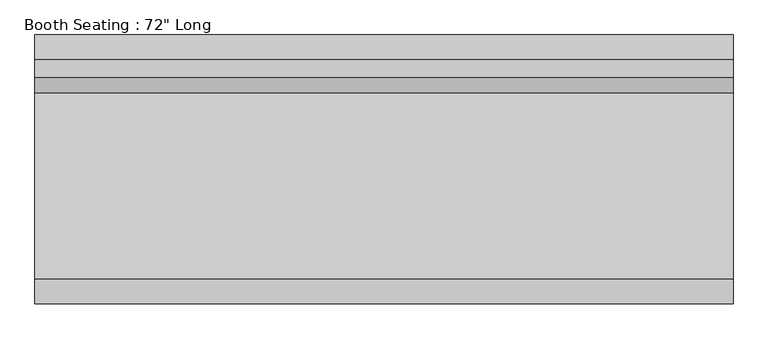
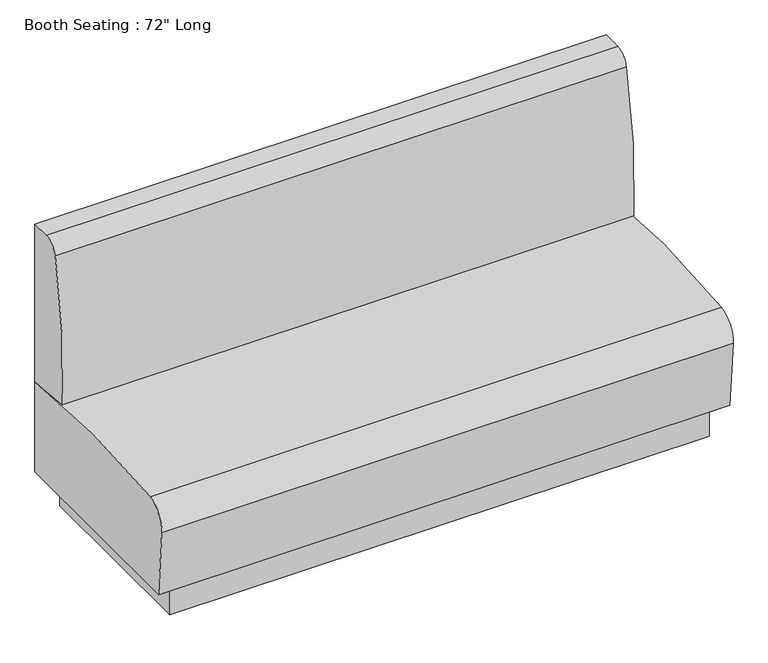
"""IFC4 building model written with IfcOpenShell, lengths in millimetres: furniture geometry."""

import ifcopenshell
import ifcopenshell.guid

model = None  # the IFC model being written
_history = None  # IfcOwnerHistory: only IFC2X3 demands one
_inside = {}  # id of a spatial element -> (the spatial element, [elements in it])
_under = {}  # id of a project, library or spatial element -> (it, [spatial elements below it])
_declared = {}  # id of a project -> (the project, [libraries it declares])
_typed = {}  # id of a type object -> (the type object, [elements of that type])
_made_of = {}  # id of a material, layer set ... -> (it, [elements and type objects made of it])


def new_model(schema):
    """Start an empty IFC model of exactly this schema.

    Asked for "IFC4X3", IfcOpenShell would pick the latest addendum, in which some entities
    have other attributes; the version numbers below select the first issue.
    IFC2X3 requires an IfcOwnerHistory on every rooted entity: one is made here for all.
    """
    global model, _history
    if schema == "IFC4X3":
        model = ifcopenshell.file(schema_version=(4, 3, 0, 0))
    else:
        model = ifcopenshell.file(schema=schema)
    _inside.clear()
    _under.clear()
    _declared.clear()
    _typed.clear()
    _made_of.clear()
    _history = None
    if model.schema == "IFC2X3":
        org = make("IfcOrganization", Name="unknown")
        user = make(
            "IfcPersonAndOrganization",
            ThePerson=make("IfcPerson", FamilyName="unknown"),
            TheOrganization=org,
        )
        app = make(
            "IfcApplication",
            ApplicationDeveloper=org,
            Version="unknown",
            ApplicationFullName="unknown",
            ApplicationIdentifier="unknown",
        )
        _history = make(
            "IfcOwnerHistory",
            OwningUser=user,
            OwningApplication=app,
            ChangeAction="ADDED",
            CreationDate=0,
        )
    return model


def make(cls, **values):
    """One entity of the class cls with the attributes given. An attribute that is None is left unset."""
    return model.create_entity(
        cls, **{name: value for name, value in values.items() if value is not None}
    )


def rooted(cls, **values):
    """An entity with a GlobalId (a new one), such as an element, a storey or a relation."""
    return make(cls, GlobalId=ifcopenshell.guid.new(), OwnerHistory=_history, **values)


def si_unit(unit_type, name, prefix=None):
    """IfcSIUnit, for example si_unit("LENGTHUNIT", "METRE", prefix="MILLI")."""
    return make("IfcSIUnit", UnitType=unit_type, Prefix=prefix, Name=name)


def assignment(units):
    """IfcUnitAssignment: the units of a project."""
    return None if units is None else make("IfcUnitAssignment", Units=units)


def point(xyz):
    """IfcCartesianPoint."""
    return None if xyz is None else make("IfcCartesianPoint", Coordinates=xyz)


def direction(xyz):
    """IfcDirection."""
    return None if xyz is None else make("IfcDirection", DirectionRatios=xyz)


def frame(location, z_axis=None, x_axis=None):
    """IfcAxis2Placement3D, a coordinate frame: its origin and axes. An axis left out is left unset."""
    return make(
        "IfcAxis2Placement3D",
        Location=point(location),
        Axis=direction(z_axis),
        RefDirection=direction(x_axis),
    )


def frame_2d(location, x_axis=None):
    """IfcAxis2Placement2D, a coordinate frame in the plane: its origin and x axis."""
    return make(
        "IfcAxis2Placement2D", Location=point(location), RefDirection=direction(x_axis)
    )


def origin():
    """The frame at (0, 0, 0) with its axes left unset."""
    return frame((0.0, 0.0, 0.0))


def origin_with_axes():
    """The frame at (0, 0, 0) with the z axis (0, 0, 1) and the x axis (1, 0, 0) written out."""
    return frame((0.0, 0.0, 0.0), z_axis=(0.0, 0.0, 1.0), x_axis=(1.0, 0.0, 0.0))


def place(relative_to, where):
    """IfcLocalPlacement: puts the frame where relative to a parent placement (None: the world)."""
    return make(
        "IfcLocalPlacement", PlacementRelTo=relative_to, RelativePlacement=where
    )


def context(
    kind, dimensions, precision=None, world=None, true_north=None, identifier=None
):
    """IfcGeometricRepresentationContext, for example the 3D "Model" context."""
    return make(
        "IfcGeometricRepresentationContext",
        ContextIdentifier=identifier,
        ContextType=kind,
        CoordinateSpaceDimension=dimensions,
        Precision=precision,
        WorldCoordinateSystem=world,
        TrueNorth=true_north,
    )


def project(units=None, contexts=None):
    """IfcProject with its units and contexts."""
    return rooted(
        "IfcProject",
        Name="project",
        RepresentationContexts=contexts,
        UnitsInContext=assignment(units),
    )


def spatial(cls, under=None, at=None, **own):
    """A site, building, storey or space (cls), placed at a placement, below another one or the project."""
    s = rooted(cls, ObjectPlacement=at, **own)
    if under is not None:
        _under.setdefault(under.id(), (under, []))[1].append(s)
    return s


def polyline(points):
    """IfcPolyline through the points."""
    return make("IfcPolyline", Points=[point(p) for p in points])


def circle_curve(where, radius):
    """IfcCircle in the frame where."""
    return make("IfcCircle", Position=where, Radius=radius)


def trimmed(basis, trim1, trim2, sense, master):
    """IfcTrimmedCurve: the piece of a basis curve between two trims."""
    return make(
        "IfcTrimmedCurve",
        BasisCurve=basis,
        Trim1=trim1,
        Trim2=trim2,
        SenseAgreement=sense,
        MasterRepresentation=master,
    )


def segment(curve, same_sense, transition):
    """IfcCompositeCurveSegment."""
    return make(
        "IfcCompositeCurveSegment",
        Transition=transition,
        SameSense=same_sense,
        ParentCurve=curve,
    )


def composite_curve(segments, self_intersect=None):
    """IfcCompositeCurve: segments joined end to end."""
    return make("IfcCompositeCurve", Segments=segments, SelfIntersect=self_intersect)


def outline(outer, holes=None, kind="AREA"):
    """IfcArbitraryClosedProfileDef: a profile drawn as a closed curve; with holes, ...WithVoids."""
    if holes is None:
        return make("IfcArbitraryClosedProfileDef", ProfileType=kind, OuterCurve=outer)
    return make(
        "IfcArbitraryProfileDefWithVoids",
        ProfileType=kind,
        OuterCurve=outer,
        InnerCurves=holes,
    )


def extrude(swept, where, along, depth):
    """IfcExtrudedAreaSolid: the profile swept, set in the frame where, extruded along a direction by depth."""
    return make(
        "IfcExtrudedAreaSolid",
        SweptArea=swept,
        Position=where,
        ExtrudedDirection=direction(along),
        Depth=depth,
    )


def shape(context_of_items, identifier, shape_type, items):
    """IfcShapeRepresentation: the items that make up one representation, for example the "Body"."""
    return make(
        "IfcShapeRepresentation",
        ContextOfItems=context_of_items,
        RepresentationIdentifier=identifier,
        RepresentationType=shape_type,
        Items=items,
    )


def source(mapping_origin, context_of_items, identifier, shape_type, items):
    """IfcRepresentationMap: a shape defined once, which mapped items show again and again."""
    return make(
        "IfcRepresentationMap",
        MappingOrigin=mapping_origin,
        MappedRepresentation=shape(context_of_items, identifier, shape_type, items),
    )


def transform(
    local_origin,
    x_axis=None,
    y_axis=None,
    z_axis=None,
    scale=None,
    scale2=None,
    scale3=None,
    uniform=True,
):
    """IfcCartesianTransformationOperator3D, or its non-uniform kind. x_axis, y_axis, z_axis: its Axis1, 2, 3."""
    if uniform:
        return make(
            "IfcCartesianTransformationOperator3D",
            Axis1=direction(x_axis),
            Axis2=direction(y_axis),
            LocalOrigin=point(local_origin),
            Scale=scale,
            Axis3=direction(z_axis),
        )
    return make(
        "IfcCartesianTransformationOperator3DnonUniform",
        Axis1=direction(x_axis),
        Axis2=direction(y_axis),
        LocalOrigin=point(local_origin),
        Scale=scale,
        Axis3=direction(z_axis),
        Scale2=scale2,
        Scale3=scale3,
    )


def mapped(mapping_source, mapping_target):
    """IfcMappedItem: shows the shape of a source again, moved by a transform."""
    return make(
        "IfcMappedItem", MappingSource=mapping_source, MappingTarget=mapping_target
    )


def made_of(thing, what):
    """Note that an element or type object is made of a material, layer set ...; save() writes the relation."""
    if what is not None:
        _made_of.setdefault(what.id(), (what, []))[1].append(thing)
    return thing


def element(
    cls,
    number,
    at=None,
    inside=None,
    cuts=None,
    type_object=None,
    material=None,
    context=None,
    identifier="Body",
    shape_type=None,
    held_by="IfcProductDefinitionShape",
    body=None,
    shapes=None,
    **own,
):
    """One element of the class cls, such as IfcWall. Its Tag is "e" and its number.

    at: its placement. inside: the storey or other place that contains it. cuts: it is an
    opening in that element (IfcRelVoidsElement). A single representation is given by context,
    identifier, shape_type and body (its items); several are given by shapes. held_by: the class
    of the entity that holds the representations. save() writes the other relations.
    """
    e = rooted(cls, Tag="e%d" % number, ObjectPlacement=at, **own)
    if body is not None:
        shapes = [shape(context, identifier, shape_type, body)]
    if shapes is not None:
        e.Representation = make(held_by, Representations=shapes)
    if inside is not None:
        _inside.setdefault(inside.id(), (inside, []))[1].append(e)
    if cuts is not None:
        rooted(
            "IfcRelVoidsElement", RelatingBuildingElement=cuts, RelatedOpeningElement=e
        )
    if type_object is not None:
        _typed.setdefault(type_object.id(), (type_object, []))[1].append(e)
    return made_of(e, material)


def aggregate(whole, parts):
    """IfcRelAggregates: a whole, such as a stair, and the parts it consists of."""
    return rooted("IfcRelAggregates", RelatingObject=whole, RelatedObjects=parts)


def save(model, path):
    """Write the relations noted so far, then the file.

    IfcRelAggregates (storeys below a building ...), IfcRelContainedInSpatialStructure (elements
    in a storey), IfcRelDefinesByType, IfcRelAssociatesMaterial and IfcRelDeclares: one each for
    every whole, place, type object, material and project.
    """
    for whole, parts in _under.values():
        aggregate(whole, parts)
    for where, things in _inside.values():
        rooted(
            "IfcRelContainedInSpatialStructure",
            RelatedElements=things,
            RelatingStructure=where,
        )
    for kind, things in _typed.values():
        rooted("IfcRelDefinesByType", RelatedObjects=things, RelatingType=kind)
    for what, things in _made_of.values():
        rooted("IfcRelAssociatesMaterial", RelatedObjects=things, RelatingMaterial=what)
    for by, libraries in _declared.values():
        rooted("IfcRelDeclares", RelatingContext=by, RelatedDefinitions=libraries)
    model.write(path)


def furniture_e9c3bc78(model_context):
    return source(origin(), model_context, "Body", "SweptSolid", [
        extrude(outline(composite_curve([segment(polyline([(355.6, 939.8), (355.6, 406.4), (203.2, 420.809063)]), True, "CONTINUOUS"), segment(trimmed(circle_curve(frame_2d((1896.6191414, 522.5154157)), 1696.4706218), [point((203.2, 420.809063))], [point((242.7504703, 900.3129667))], False, "CARTESIAN"), True, "CONTINUOUS"), segment(trimmed(circle_curve(frame_2d((292.2747753, 889.0)), 50.8), [point((242.7504703, 900.3129667))], [point((292.2747753, 939.8))], False, "CARTESIAN"), True, "CONTINUOUS"), segment(polyline([(292.2747753, 939.8), (355.6, 939.8)]), True, "CONTINUOUS")], self_intersect=False)), frame((-914.4, 0.0, 0.0), z_axis=(1.0, 0.0, 0.0), x_axis=(0.0, 1.0, 0.0)), (0.0, 0.0, 1.0), 1828.8),
        extrude(outline(composite_curve([segment(trimmed(circle_curve(frame_2d((-272.6641824, 328.7396957)), 76.2), [point((-348.6009692, 322.4116302))], [point((-282.6626275, 404.2808838))], False, "CARTESIAN"), True, "CONTINUOUS"), segment(trimmed(circle_curve(frame_2d((44.6835428, -2068.9155338)), 2494.7657275), [point((-282.6626275, 404.2808838))], [point((355.6, 406.4))], False, "CARTESIAN"), True, "CONTINUOUS"), segment(polyline([(355.6, 406.4), (355.6, 101.6), (-330.2, 101.6), (-348.6009692, 322.4116302)]), True, "CONTINUOUS")], self_intersect=False)), frame((-914.4, 0.0, 0.0), z_axis=(1.0, 0.0, 0.0), x_axis=(0.0, 1.0, 0.0)), (0.0, 0.0, 1.0), 1828.8),
        extrude(outline(polyline([(863.6, 304.8), (863.6, -304.8), (-863.6, -304.8), (-863.6, 304.8), (863.6, 304.8)])), origin_with_axes(), (0.0, 0.0, 1.0), 101.6),
    ])


if __name__ == "__main__":
    model = new_model("IFC4")
    model_context = context("Model", 3, world=origin())
    ifc_project = project(units=[si_unit("LENGTHUNIT", "METRE", prefix="MILLI")], contexts=[model_context])
    site = spatial("IfcSite", under=ifc_project)
    building = spatial("IfcBuilding", under=site)
    placement = place(None, origin())
    furniture_shape = furniture_e9c3bc78(model_context)
    element("IfcFurniture", 1, ObjectType="Booth Seating : 72\" Long", at=placement, inside=building, context=model_context, shape_type="MappedRepresentation", body=[
        mapped(furniture_shape, transform((0.0, 0.0, 0.0), x_axis=(1.0, 0.0, 0.0), y_axis=(0.0, 1.0, 0.0), z_axis=(0.0, 0.0, 1.0))),
    ])
    save(model, "model.ifc")

# Revit data of these elements
# Project information
#   Project Issue Date = "Issue Date"
#   Project Status = "Project Status"
#   Client Name = "Owner"
#   Project Address = "Enter address here"
#   Project Name = "Project Name"
#   Project Number = "Project Number"
# Type "Booth Seating : 72\" Long"
#   Seat Height = 1' - 4"
#   Length = 6' - 0"
#   Depth = 2' - 4"
#   Back Height = 3' - 1"
#   Default Elevation = 0
# Element 1 (IfcFurniture, "Booth Seating : 72\" Long")
#   Materials on its faces: "Leather, Dark Brown", "Plastic, Opaque Black"
# Materials
#   "Leather, Dark Brown": class "Textile", colour RGB 57 45 39, transparency 0, Description = "Leather, dark brown", Cost = 0
#   "Plastic, Opaque Black": class "Plastic", colour RGB 5 5 5, transparency 0, Description = "Plastic, generic, opaque black", Cost = 0
